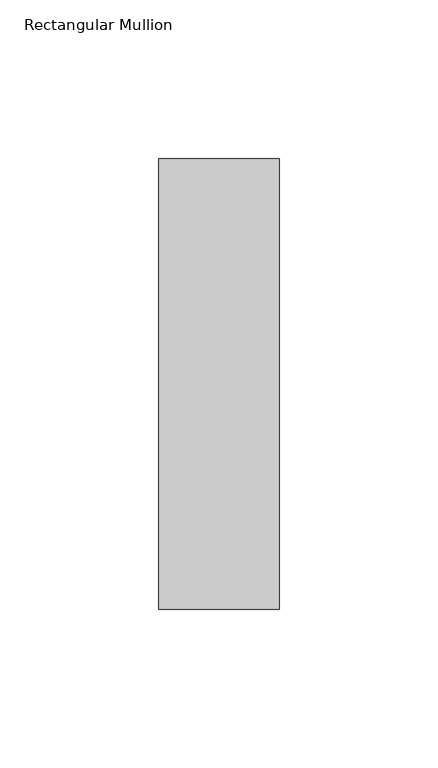
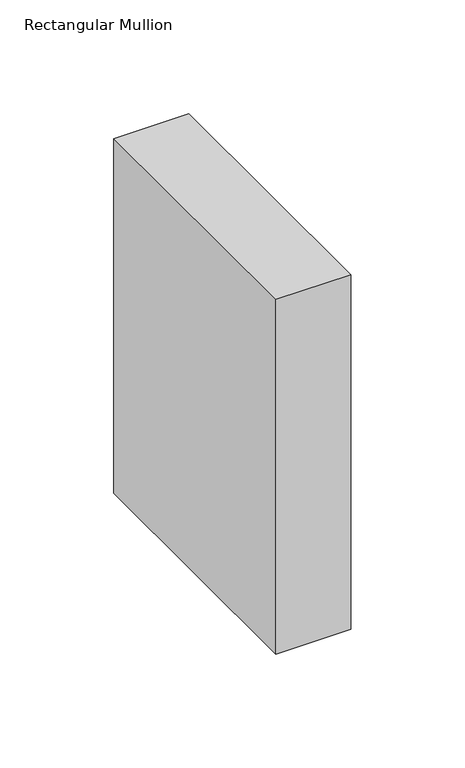
"""IFC4 building model written with IfcOpenShell, lengths in millimetres: member geometry, Rectangular Mullion : NLRS_21_CWM_hsb-regel 38x142_gen_rsf."""

from ifc_helpers import new_model, si_unit, frame, origin, place, context, project, spatial, polyline, outline, extrude, source, transform, mapped, element, save


def rectangular_mullion_07180aef(model_context):
    return source(origin(), model_context, "Body", "SweptSolid", [
        extrude(outline(polyline([(-38.0, -71.0), (-38.0, 71.0), (0.0, 71.0), (0.0, -71.0), (-38.0, -71.0)])), frame((0.0, 0.0, -189.9999997), z_axis=(0.0, 0.0, 1.0), x_axis=(1.0, 0.0, 0.0)), (0.0, 0.0, 1.0), 189.9999997),
    ])


if __name__ == "__main__":
    model = new_model("IFC4")
    model_context = context("Model", 3, world=origin())
    ifc_project = project(units=[si_unit("LENGTHUNIT", "METRE", prefix="MILLI")], contexts=[model_context])
    site = spatial("IfcSite", under=ifc_project)
    building = spatial("IfcBuilding", under=site)
    placement = place(None, origin())
    rectangular_mullion_shape = rectangular_mullion_07180aef(model_context)
    element("IfcMember", 1, ObjectType="Rectangular Mullion : NLRS_21_CWM_hsb-regel 38x142_gen_rsf", at=placement, inside=building, context=model_context, shape_type="MappedRepresentation", body=[
        mapped(rectangular_mullion_shape, transform((0.0, 0.0, 0.0), x_axis=(1.0, 0.0, 0.0), y_axis=(0.0, 1.0, 0.0), z_axis=(0.0, 0.0, 1.0))),
    ])
    save(model, "model.ifc")

# Revit data of these elements
# Type "Rectangular Mullion : NLRS_21_CWM_hsb-regel 38x142_gen_rsf"
#   Export Type to IFC As = "IfcWall"
#   Type IfcGUID = "07M7mRoiH1CR8m_RSKIwpF"
#   Assembly Code = "21.10"
#   built-in parameter 1007322 = 0.465879 (stored number, unit not read)
#   built-in parameter 1007321 = 0.062336 (stored number, unit not read)
#   built-in parameter 1007320 = 0.062336 (stored number, unit not read)
# Element 1 (IfcMember, "Rectangular Mullion : NLRS_21_CWM_hsb-regel 38x142_gen_rsf")
#   Materials on its faces: "NLRS_i2_hout naaldhout vuren_gen_rsf"
# Materials
#   "NLRS_i2_hout naaldhout vuren_gen_rsf": class "I - Hout", colour RGB 234 199 147, transparency 0, Keynote = "i2", Manufacturer = "Revit Standards Foundation", URL = "www.revitstandards.org", Description = "hout vuren", Cost = 0
